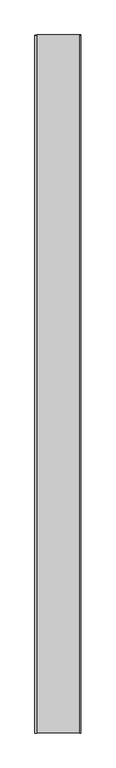
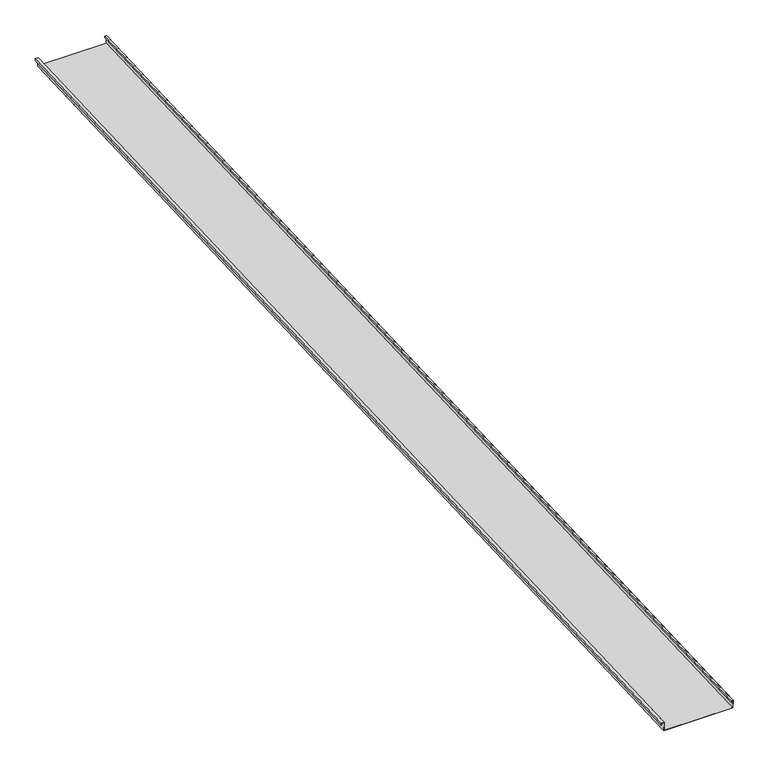
"""IFC4 building model written with IfcOpenShell, lengths in millimetres: proxy geometry, Generic Models 2:Generic Models 2:310765:Generic Models 2:310765 : Generic Models 2:Generic Models 2:310765:115 : Generic Models 2:Generic Models 2:310765:Generic Models 2:310765 : Generic Models 2:Generic Models 2:310765:300385."""

from ifc_helpers import new_model, si_unit, frame, origin, place, context, project, spatial, polyline, outline, extrude, source, transform, mapped, element, save


def generic_models_f714f371(model_context):
    return source(origin(), model_context, "Body", "SweptSolid", [
        extrude(outline(polyline([(1.5875, 0.0), (1.5875, 50.8), (407.9875, 50.8), (407.9875, 1.5875), (396.875, 1.5875), (396.875, 11.1125), (398.4625, 11.1125), (398.4625, 3.175), (406.4, 3.175), (406.4, 49.2125), (3.175, 49.2125), (3.175, -1.5874999), (-14.2875, -1.5874999), (-14.2875, 9.525), (-12.7, 9.525), (-12.7, 0.0), (1.5875, 0.0)])), frame((666660.6929738, -581354.4345603, 3902.6697972), z_axis=(0.0, 0.9991330730923568, 0.041630544712067834), x_axis=(1.0, 0.0, 0.0)), (0.0, 0.0, 1.0), 6400.8),
    ])


if __name__ == "__main__":
    model = new_model("IFC4")
    model_context = context("Model", 3, world=origin())
    ifc_project = project(units=[si_unit("LENGTHUNIT", "METRE", prefix="MILLI")], contexts=[model_context])
    site = spatial("IfcSite", under=ifc_project)
    building = spatial("IfcBuilding", under=site)
    placement = place(None, origin())
    generic_models_shape = generic_models_f714f371(model_context)
    element("IfcBuildingElementProxy", 1, Name="Generic Models 2:Generic Models 2:310765:Generic Models 2:310765 : Generic Models 2:Generic Models 2:310765:115 : Generic Models 2:Generic Models 2:310765:Generic Models 2:310765 : Generic Models 2:Generic Models 2:310765:300385", ObjectType="Generic Models 2:Generic Models 2:310765:Generic Models 2:310765 : Generic Models 2:Generic Models 2:310765:115 : Generic Models 2:Generic Models 2:310765:Generic Models 2:310765 : Generic Models 2:Generic Models 2:310765:300385", at=placement, inside=building, context=model_context, shape_type="MappedRepresentation", body=[
        mapped(generic_models_shape, transform((0.0, 0.0, 0.0), x_axis=(1.0, 0.0, 0.0), y_axis=(0.0, 1.0, 0.0), z_axis=(0.0, 0.0, 1.0))),
    ])
    save(model, "model.ifc")

# Revit data of these elements
# Type "Generic Models 2:Generic Models 2:310765:Generic Models 2:310765 : Generic Models 2:Generic Models 2:310765:115 : Generic Models 2:Generic Models 2:310765:Generic Models 2:310765 : Generic Models 2:Generic Models 2:310765:300385"
#   NameOverride = "Generic Models 2:Generic Models 2:310765:Generic Models 2:310765 : Generic Models 2:Generic Models 2:310765:300385"
#   ObjectTypeOverride = "Generic Models 2:310765 : Generic Models 2:Generic Models 2:310765"
#   Reference = "Generic Models 2"
#   Tag = "300385"
# Element 1 (IfcBuildingElementProxy, "Generic Models 2:Generic Models 2:310765:Generic Models 2:310765 : Generic Models 2:Generic Models 2:310765:115 : Generic Models 2:Generic Models 2:310765:Generic Models 2:310765 : Generic Models 2:Generic Models 2:310765:300385")
#   Materials on its faces: "THERMAL BROKEN ALUMINUM STOREFRONT FOR POLYCARBONATE"
# Materials
#   "THERMAL BROKEN ALUMINUM STOREFRONT FOR POLYCARBONATE": class "Unassigned", colour RGB 244 244 244, transparency 0, Keynote = "M07611300.01", Cost = 0
